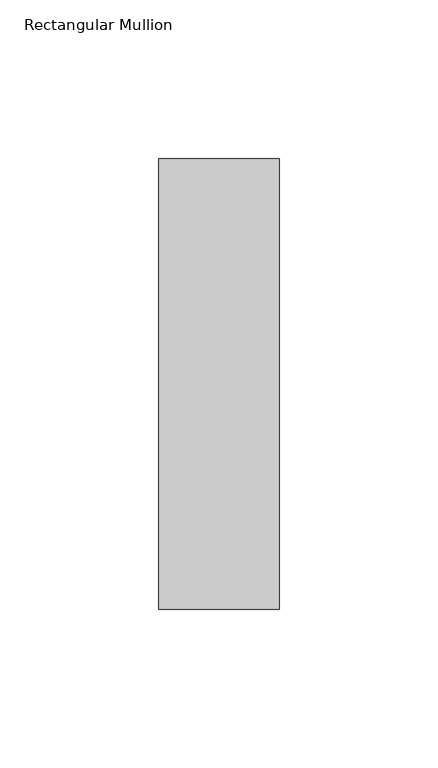
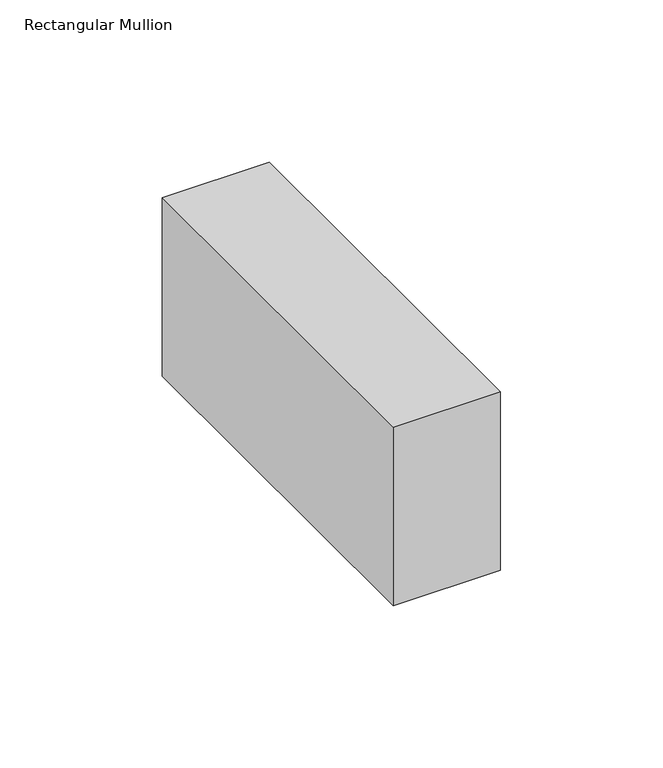
"""IFC4 building model written with IfcOpenShell, lengths in millimetres: member geometry, Rectangular Mullion : NLRS_21_CWM_hsb-regel 38x142_gen_rsf."""

from ifc_helpers import new_model, si_unit, frame, origin, place, context, project, spatial, polyline, outline, extrude, source, transform, mapped, element, save


def rectangular_mullion_f185e772(model_context):
    return source(origin(), model_context, "Body", "SweptSolid", [
        extrude(outline(polyline([(0.0, -71.0), (-38.0, -71.0), (-38.0, 71.0), (0.0, 71.0), (0.0, -71.0)])), frame((0.0, 0.0, -66.9999997), z_axis=(0.0, 0.0, 1.0), x_axis=(1.0, 0.0, 0.0)), (0.0, 0.0, 1.0), 66.9999997),
    ])


if __name__ == "__main__":
    model = new_model("IFC4")
    model_context = context("Model", 3, world=origin())
    ifc_project = project(units=[si_unit("LENGTHUNIT", "METRE", prefix="MILLI")], contexts=[model_context])
    site = spatial("IfcSite", under=ifc_project)
    building = spatial("IfcBuilding", under=site)
    placement = place(None, origin())
    rectangular_mullion_shape = rectangular_mullion_f185e772(model_context)
    element("IfcMember", 1, ObjectType="Rectangular Mullion : NLRS_21_CWM_hsb-regel 38x142_gen_rsf", at=placement, inside=building, context=model_context, shape_type="MappedRepresentation", body=[
        mapped(rectangular_mullion_shape, transform((0.0, 0.0, 0.0), x_axis=(1.0, 0.0, 0.0), y_axis=(0.0, 1.0, 0.0), z_axis=(0.0, 0.0, 1.0))),
    ])
    save(model, "model.ifc")

# Revit data of these elements
# Type "Rectangular Mullion : NLRS_21_CWM_hsb-regel 38x142_gen_rsf"
#   Export Type to IFC As = "IfcWall"
#   Type IfcGUID = "07M7mRoiH1CR8m_RSKIwpF"
#   Assembly Code = "21.10"
#   built-in parameter 1007322 = 0.465879 (stored number, unit not read)
#   built-in parameter 1007321 = 0.062336 (stored number, unit not read)
#   built-in parameter 1007320 = 0.062336 (stored number, unit not read)
# Element 1 (IfcMember, "Rectangular Mullion : NLRS_21_CWM_hsb-regel 38x142_gen_rsf")
#   Materials on its faces: "NLRS_i2_hout naaldhout vuren_gen_rsf"
# Materials
#   "NLRS_i2_hout naaldhout vuren_gen_rsf": class "I - Hout", colour RGB 234 199 147, transparency 0, Keynote = "i2", Manufacturer = "Revit Standards Foundation", URL = "www.revitstandards.org", Description = "hout vuren", Cost = 0
